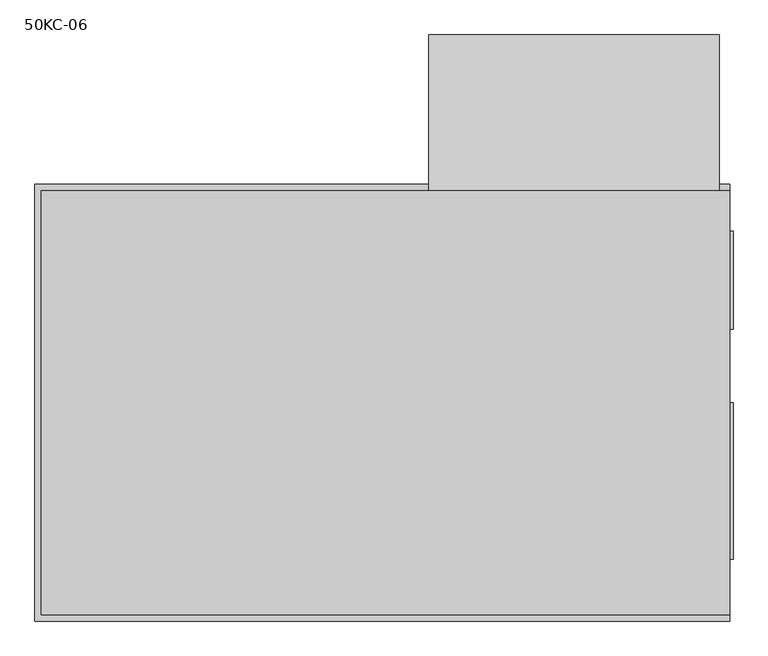
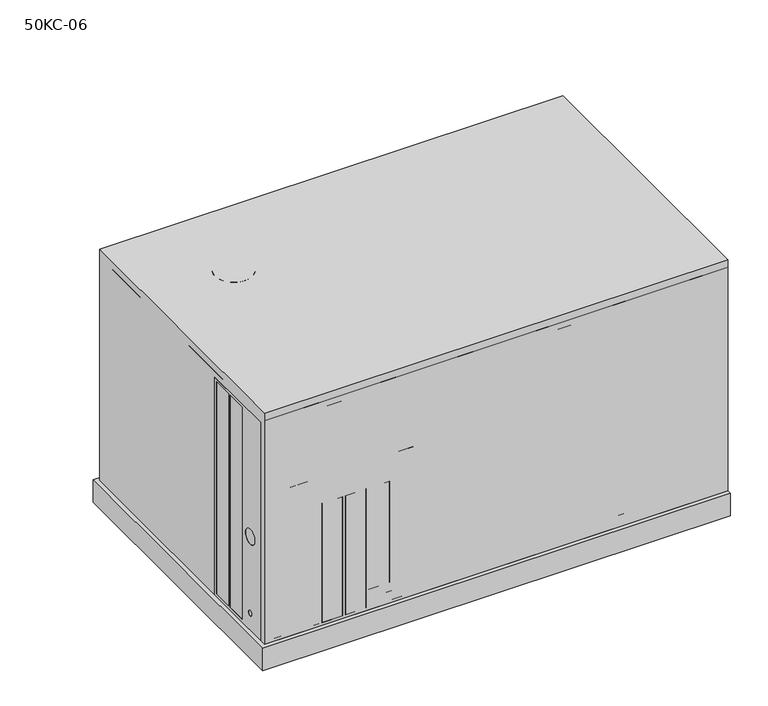
"""IFC4 building model written with IfcOpenShell, lengths in millimetres: proxy geometry, AHU-Rooftop-Carrier-Cooling_&_Elec_Heating-3-5_ton : 50KC-06."""

from ifc_helpers import new_model, si_unit, point, frame, frame_2d, origin, origin_with_axes, place, context, project, spatial, polyline, circle_curve, trimmed, segment, composite_curve, outline, extrude, faceted_brep, source, transform, mapped, element, save
from ifc_brep_helpers import plane_surface, cylinder_surface, revolved_surface, advanced_brep


def proxy_50kc_06_755dc8fb(model_context):
    return source(origin(), model_context, "Body", "SolidModel", [
        extrude(outline(polyline([(-547.6875, 1025.525), (-228.6, 1025.525), (-228.6, 95.25), (-547.6875, 95.25), (-547.6875, 1025.525)]), holes=[polyline([(-323.85, 1012.825), (-323.85, 107.95), (-241.3, 107.95), (-241.3, 1012.825), (-323.85, 1012.825)]), polyline([(-419.1, 1012.825), (-419.1, 107.95), (-336.55, 107.95), (-336.55, 1012.825), (-419.1, 1012.825)]), composite_curve([segment(trimmed(circle_curve(frame_2d((-476.25, 495.3)), 31.75), [point((-508.0, 495.3))], [point((-444.5, 495.3))], True, "CARTESIAN"), True, "CONTINUOUS"), segment(trimmed(circle_curve(frame_2d((-476.25, 495.3)), 31.75), [point((-444.5, 495.3))], [point((-508.0, 495.3))], True, "CARTESIAN"), True, "CONTINUOUS")], self_intersect=False), composite_curve([segment(trimmed(circle_curve(frame_2d((-476.25, 168.275)), 11.1125), [point((-487.3625, 168.275))], [point((-465.1375, 168.275))], True, "CARTESIAN"), True, "CONTINUOUS"), segment(trimmed(circle_curve(frame_2d((-476.25, 168.275)), 11.1125), [point((-465.1375, 168.275))], [point((-487.3625, 168.275))], True, "CARTESIAN"), True, "CONTINUOUS")], self_intersect=False)]), frame((-927.1, 0.0, 0.0), z_axis=(1.0, 0.0, 0.0), x_axis=(0.0, 1.0, 0.0)), (0.0, 0.0, 1.0), 3.175),
        advanced_brep(
        [(941.3875, 573.0875, 1025.525), (-436.5625, 573.0875, 1025.525), (-436.5625, 534.9875, 1025.525), (-885.825, 534.9875, 1025.525), (-885.825, -215.9, 1025.525), (-923.925, -215.9, 1025.525), (-923.925, -573.0875, 1025.525), (941.3875, -573.0875, 1025.525), (-883.285, 532.4475, 1025.525), (-436.5625, 532.4475, 1025.525), (-436.5625, -215.9, 1025.525), (-883.285, -215.9, 1025.525), (941.3875, 573.0875, 95.25), (941.3875, -573.0875, 95.25), (-923.925, -573.0875, 95.25), (-923.925, -215.9, 95.25), (-885.825, -215.9, 95.25), (-885.825, 534.9875, 95.25), (-436.5625, 534.9875, 95.25), (-436.5625, 573.0875, 95.25), (-883.285, 532.4475, 95.25), (-883.285, -215.9, 95.25), (-436.5625, -215.9, 95.25), (-436.5625, 532.4475, 95.25), (-923.925, -508.0, 495.3), (-923.925, -444.5, 495.3), (-923.925, -487.3625, 168.275), (-923.925, -465.1375, 168.275), (941.3875, 88.9, 194.1909375), (941.3875, 88.9, 161.4090625), (919.1625, 88.9, 161.4090625), (919.1625, 88.9, 194.1909375), (-914.4, -508.0, 495.3), (-914.4, -444.5, 495.3), (-914.4, -487.3625, 168.275), (-914.4, -465.1375, 168.275)],
        [
            (0, 1),
            (1, 2),
            (2, 3),
            (3, 4),
            (4, 5),
            (5, 6),
            (6, 7),
            (7, 0),
            (8, 9),
            (9, 10),
            (10, 11),
            (11, 8),
            (12, 13),
            (13, 14),
            (14, 15),
            (15, 16),
            (16, 17),
            (17, 18),
            (18, 19),
            (19, 12),
            (20, 21),
            (21, 22),
            (22, 23),
            (23, 20),
            (0, 12),
            (19, 1),
            (5, 15),
            (14, 6),
            (24, 25, circle_curve(frame((-923.925, -476.25, 495.3), z_axis=(1.0, 0.0, 0.0), x_axis=(0.0, 1.0, 0.0)), 31.75)),
            (25, 24, circle_curve(frame((-923.925, -476.25, 495.3), z_axis=(1.0, 0.0, 0.0), x_axis=(0.0, 1.0, 0.0)), 31.75)),
            (26, 27, circle_curve(frame((-923.925, -476.25, 168.275), z_axis=(1.0, 0.0, 0.0), x_axis=(0.0, 1.0, 0.0)), 11.1125)),
            (27, 26, circle_curve(frame((-923.925, -476.25, 168.275), z_axis=(1.0, 0.0, 0.0), x_axis=(0.0, 1.0, 0.0)), 11.1125)),
            (13, 7),
            (28, 29, circle_curve(frame((941.3875, 88.9, 177.8), z_axis=(-1.0, 0.0, 0.0), x_axis=(0.0, 0.0, 1.0)), 16.3909375)),
            (29, 28, circle_curve(frame((941.3875, 88.9, 177.8), z_axis=(-1.0, 0.0, 0.0), x_axis=(0.0, 0.0, 1.0)), 16.3909375)),
            (18, 2),
            (17, 3),
            (16, 4),
            (30, 31, circle_curve(frame((919.1625, 88.9, 177.8), z_axis=(1.0, 0.0, 0.0), x_axis=(0.0, 0.0, 1.0)), 16.3909375)),
            (31, 30, circle_curve(frame((919.1625, 88.9, 177.8), z_axis=(1.0, 0.0, 0.0), x_axis=(0.0, 0.0, 1.0)), 16.3909375)),
            (30, 29),
            (28, 31),
            (32, 33, circle_curve(frame((-914.4, -476.25, 495.3), z_axis=(-1.0, 0.0, 0.0), x_axis=(0.0, 1.0, 0.0)), 31.75)),
            (33, 32, circle_curve(frame((-914.4, -476.25, 495.3), z_axis=(-1.0, 0.0, 0.0), x_axis=(0.0, 1.0, 0.0)), 31.75)),
            (34, 35, circle_curve(frame((-914.4, -476.25, 168.275), z_axis=(-1.0, 0.0, 0.0), x_axis=(0.0, 1.0, 0.0)), 11.1125)),
            (35, 34, circle_curve(frame((-914.4, -476.25, 168.275), z_axis=(-1.0, 0.0, 0.0), x_axis=(0.0, 1.0, 0.0)), 11.1125)),
            (33, 25),
            (24, 32),
            (35, 27),
            (26, 34),
            (8, 20),
            (23, 9),
            (22, 10),
            (21, 11),
        ],
        [
            plane_surface(frame((-466.3462048, 573.0875, 1025.525), z_axis=(0.0, 0.0, 1.0), x_axis=(-1.0, 0.0, 0.0))),
            plane_surface(frame((-466.3462048, 573.0875, 95.25), z_axis=(0.0, 0.0, -1.0), x_axis=(1.0, 0.0, 0.0))),
            plane_surface(frame((941.3875, 573.0875, 1025.525), z_axis=(0.0, 1.0, 0.0), x_axis=(0.0, 0.0, -1.0))),
            plane_surface(frame((-923.925, -215.9, 1025.525), z_axis=(-1.0, 0.0, 0.0), x_axis=(0.0, 0.0, -1.0))),
            plane_surface(frame((-923.925, -573.0875, 1025.525), z_axis=(0.0, -1.0, 0.0), x_axis=(0.0, 0.0, -1.0))),
            plane_surface(frame((941.3875, -573.0875, 1025.525), z_axis=(1.0, 0.0, 0.0), x_axis=(0.0, 0.0, -1.0))),
            plane_surface(frame((-436.5625, 573.0875, 1025.525), z_axis=(-1.0, 0.0, 0.0), x_axis=(0.0, 0.0, -1.0))),
            plane_surface(frame((-436.5625, 534.9875, 1025.525), z_axis=(0.0, 1.0, 0.0), x_axis=(0.0, 0.0, -1.0))),
            plane_surface(frame((-885.825, 534.9875, 1025.525), z_axis=(-1.0, 0.0, 0.0), x_axis=(0.0, 0.0, -1.0))),
            plane_surface(frame((-885.825, -215.9, 1025.525), z_axis=(0.0, 1.0, 0.0), x_axis=(0.0, 0.0, -1.0))),
            plane_surface(frame((919.1625, 88.9, 177.8), z_axis=(1.0, 0.0, 0.0), x_axis=(0.0, 1.0, 0.0))),
            revolved_surface(polyline([(941.3875, 88.9, 194.19093750000002), (919.1625, 88.9, 194.19093750000002)]), (944.5625, 88.9, 177.8), (1.0, 0.0, 0.0)),
            plane_surface(frame((-914.4, -444.5, 495.3), z_axis=(-1.0, 0.0, 0.0), x_axis=(0.0, 0.0, 1.0))),
            revolved_surface(polyline([(-914.4, -444.5, 495.3), (-923.925, -444.5, 495.3)]), (-927.1, -476.25, 495.3), (1.0, 0.0, 0.0)),
            revolved_surface(polyline([(-914.4, -465.1375, 168.275), (-923.925, -465.1375, 168.275)]), (-927.1, -476.25, 168.275), (1.0, 0.0, 0.0)),
            plane_surface(frame((-883.285, 532.4475, 1025.525), z_axis=(0.0, -1.0, 0.0), x_axis=(0.0, 0.0, -1.0))),
            plane_surface(frame((-436.5625, 532.4475, 1025.525), z_axis=(-1.0, 0.0, 0.0), x_axis=(0.0, 0.0, -1.0))),
            plane_surface(frame((-436.5625, -215.9, 1025.525), z_axis=(0.0, 1.0, 0.0), x_axis=(0.0, 0.0, -1.0))),
            plane_surface(frame((-883.285, -215.9, 1025.525), z_axis=(1.0, 0.0, 0.0), x_axis=(0.0, 0.0, -1.0))),
        ],
        [
            (0, [[1, 2, 3, 4, 5, 6, 7, 8], [9, 10, 11, 12]]),
            (1, [[13, 14, 15, 16, 17, 18, 19, 20], [21, 22, 23, 24]]),
            (2, [[-1, 25, -20, 26]]),
            (3, [[-6, 27, -15, 28], [29, 30], [31, 32]]),
            (4, [[-7, -28, -14, 33]]),
            (5, [[-8, -33, -13, -25], [34, 35]]),
            (6, [[-2, -26, -19, 36]]),
            (7, [[-3, -36, -18, 37]]),
            (8, [[-4, -37, -17, 38]]),
            (9, [[-5, -38, -16, -27]]),
            (10, [[39, 40]]),
            (11, [[-39, 41, -34, 42]]),
            (11, [[-40, -42, -35, -41]]),
            (12, [[43, 44]]),
            (12, [[45, 46]]),
            (13, [[-44, 47, -29, 48]]),
            (13, [[-43, -48, -30, -47]]),
            (14, [[-46, 49, -31, 50]]),
            (14, [[-45, -50, -32, -49]]),
            (15, [[-9, 51, -24, 52]]),
            (16, [[-10, -52, -23, 53]]),
            (17, [[-11, -53, -22, 54]]),
            (18, [[-12, -54, -21, -51]]),
        ],
    ),
        faceted_brep([(-898.525, 573.0875, 1025.525), (-923.925, 573.0875, 1025.525), (-923.925, 547.6875, 1025.525), (-898.525, 547.6875, 1025.525), (-898.525, 573.0875, 95.25), (-898.525, 547.6875, 95.25), (-923.925, 547.6875, 95.25), (-923.925, 573.0875, 95.25)], [[[0, 1, 2, 3]], [[4, 5, 6, 7]], [[1, 0, 4, 7]], [[2, 1, 7, 6]], [[3, 2, 6, 5]], [[0, 3, 5, 4]]]),
        extrude(outline(polyline([(941.3875, 466.725), (954.0875, 466.725), (954.0875, 200.025), (941.3875, 200.025), (941.3875, 466.725)])), frame((0.0, 0.0, 155.575), z_axis=(0.0, 0.0, 1.0), x_axis=(1.0, 0.0, 0.0)), (0.0, 0.0, 1.0), 638.175),
        extrude(outline(polyline([(941.3875, 0.0), (954.0875, 0.0), (954.0875, -425.45), (941.3875, -425.45), (941.3875, 0.0)])), frame((0.0, 0.0, 155.575), z_axis=(0.0, 0.0, 1.0), x_axis=(1.0, 0.0, 0.0)), (0.0, 0.0, 1.0), 288.925),
        extrude(outline(polyline([(944.5625, 576.2625), (944.5625, -576.2625), (-927.1, -576.2625), (-927.1, 576.2625), (944.5625, 576.2625)])), frame((0.0, 0.0, 95.25), z_axis=(0.0, 0.0, 1.0), x_axis=(1.0, 0.0, 0.0)), (0.0, 0.0, 1.0), 987.425),
        extrude(outline(polyline([(-944.5625, 593.725), (944.5625, 593.725), (944.5625, -593.725), (-944.5625, -593.725), (-944.5625, 593.725)])), origin_with_axes(), (0.0, 0.0, 1.0), 95.25),
        extrude(outline(polyline([(21.43125, -576.2625), (-3.96875, -576.2625), (-3.96875, 576.2625), (21.43125, 576.2625), (21.43125, -576.2625)])), frame((0.0, 0.0, 1050.925), z_axis=(0.0, 0.0, 1.0), x_axis=(1.0, 0.0, 0.0)), (0.0, 0.0, 1.0), 12.7),
        extrude(outline(polyline([(1025.525, -411.1625), (95.25, -411.1625), (95.25, 101.6), (1025.525, 101.6), (1025.525, -411.1625)]), holes=[polyline([(177.8, -202.40625), (177.8, -107.15625), (146.05, -107.15625), (146.05, -202.40625), (177.8, -202.40625)])]), frame((0.0, 573.0875, 0.0), z_axis=(0.0, 1.0, 0.0), x_axis=(0.0, 0.0, 1.0)), (0.0, 0.0, 1.0), 3.175),
        extrude(outline(polyline([(915.9875, 573.0875), (127.0, 573.0875), (127.0, 576.2625), (915.9875, 576.2625), (915.9875, 573.0875)])), frame((0.0, 0.0, 546.1), z_axis=(0.0, 0.0, 1.0), x_axis=(1.0, 0.0, 0.0)), (0.0, 0.0, 1.0), 479.425),
        extrude(outline(polyline([(915.9875, 573.0875), (127.0, 573.0875), (127.0, 576.2625), (915.9875, 576.2625), (915.9875, 573.0875)])), frame((0.0, 0.0, 95.25), z_axis=(0.0, 0.0, 1.0), x_axis=(1.0, 0.0, 0.0)), (0.0, 0.0, 1.0), 444.5),
        extrude(outline(polyline([(-923.925, -336.55), (-923.925, -419.1), (-927.1, -419.1), (-927.1, -336.55), (-923.925, -336.55)])), frame((0.0, 0.0, 107.95), z_axis=(0.0, 0.0, 1.0), x_axis=(1.0, 0.0, 0.0)), (0.0, 0.0, 1.0), 904.875),
        extrude(outline(polyline([(-923.925, -241.3), (-923.925, -323.85), (-927.1, -323.85), (-927.1, -241.3), (-923.925, -241.3)])), frame((0.0, 0.0, 107.95), z_axis=(0.0, 0.0, 1.0), x_axis=(1.0, 0.0, 0.0)), (0.0, 0.0, 1.0), 904.875),
        extrude(outline(polyline([(-803.275, -576.2625), (-885.825, -576.2625), (-885.825, -573.0875), (-803.275, -573.0875), (-803.275, -576.2625)])), frame((0.0, 0.0, 107.95), z_axis=(0.0, 0.0, 1.0), x_axis=(1.0, 0.0, 0.0)), (0.0, 0.0, 1.0), 622.3),
        extrude(outline(polyline([(-708.025, -576.2625), (-790.575, -576.2625), (-790.575, -573.0875), (-708.025, -573.0875), (-708.025, -576.2625)])), frame((0.0, 0.0, 107.95), z_axis=(0.0, 0.0, 1.0), x_axis=(1.0, 0.0, 0.0)), (0.0, 0.0, 1.0), 622.3),
        extrude(outline(polyline([(-612.775, -576.2625), (-695.325, -576.2625), (-695.325, -573.0875), (-612.775, -573.0875), (-612.775, -576.2625)])), frame((0.0, 0.0, 107.95), z_axis=(0.0, 0.0, 1.0), x_axis=(1.0, 0.0, 0.0)), (0.0, 0.0, 1.0), 508.0),
        extrude(outline(polyline([(-517.525, -576.2625), (-600.075, -576.2625), (-600.075, -573.0875), (-517.525, -573.0875), (-517.525, -576.2625)])), frame((0.0, 0.0, 107.95), z_axis=(0.0, 0.0, 1.0), x_axis=(1.0, 0.0, 0.0)), (0.0, 0.0, 1.0), 508.0),
        extrude(outline(polyline([(-422.275, -576.2625), (-504.825, -576.2625), (-504.825, -573.0875), (-422.275, -573.0875), (-422.275, -576.2625)])), frame((0.0, 0.0, 184.15), z_axis=(0.0, 0.0, 1.0), x_axis=(1.0, 0.0, 0.0)), (0.0, 0.0, 1.0), 431.8),
        extrude(outline(polyline([(-327.025, -576.2625), (-409.575, -576.2625), (-409.575, -573.0875), (-327.025, -573.0875), (-327.025, -576.2625)])), frame((0.0, 0.0, 107.95), z_axis=(0.0, 0.0, 1.0), x_axis=(1.0, 0.0, 0.0)), (0.0, 0.0, 1.0), 622.3),
        extrude(outline(polyline([(1025.525, 915.9875), (1025.525, 34.13125), (95.25, 34.13125), (95.25, 915.9875), (1025.525, 915.9875)]), holes=[polyline([(177.8, 522.684375), (146.05, 522.684375), (146.05, 427.434375), (177.8, 427.434375), (177.8, 522.684375)])]), frame((0.0, -576.2625, 0.0), z_axis=(0.0, 1.0, 0.0), x_axis=(0.0, 0.0, 1.0)), (0.0, 0.0, 1.0), 3.175),
        extrude(outline(polyline([(1025.525, -16.66875), (1025.525, -898.525), (95.25, -898.525), (95.25, -16.66875), (1025.525, -16.66875)]), holes=[polyline([(177.8, -415.925), (146.05, -415.925), (146.05, -511.175), (177.8, -511.175), (177.8, -415.925)]), polyline([(730.25, -803.275), (107.95, -803.275), (107.95, -885.825), (730.25, -885.825), (730.25, -803.275)]), polyline([(730.25, -708.025), (107.95, -708.025), (107.95, -790.575), (730.25, -790.575), (730.25, -708.025)]), polyline([(615.95, -612.775), (107.95, -612.775), (107.95, -695.325), (615.95, -695.325), (615.95, -612.775)]), polyline([(615.95, -517.525), (107.95, -517.525), (107.95, -600.075), (615.95, -600.075), (615.95, -517.525)]), polyline([(615.95, -422.275), (184.15, -422.275), (184.15, -504.825), (615.95, -504.825), (615.95, -422.275)]), polyline([(730.25, -327.025), (107.95, -327.025), (107.95, -409.575), (730.25, -409.575), (730.25, -327.025)])]), frame((0.0, -576.2625, 0.0), z_axis=(0.0, 1.0, 0.0), x_axis=(0.0, 0.0, 1.0)), (0.0, 0.0, 1.0), 3.175),
        extrude(outline(polyline([(1000.125, 464.451767), (997.9196681, 451.9447085), (947.8914343, 460.7660359), (709.1843069, 119.8569277), (573.0875, 107.95), (573.0875, 539.75), (1000.125, 464.451767)])), frame((127.0, 0.0, 0.0), z_axis=(1.0, 0.0, 0.0), x_axis=(0.0, 1.0, 0.0)), (0.0, 0.0, 1.0), 788.9875),
        advanced_brep(
        [(-584.2, 233.3625, 1082.675), (-660.4, 233.3625, 1082.675), (-508.0, 233.3625, 1082.675), (-660.4, 233.3625, 1079.5), (-508.0, 233.3625, 1079.5), (-863.6, 233.3625, 1050.925), (-304.8, 233.3625, 1050.925), (-584.2, 233.3625, 1050.925)],
        [
            (0, 1),
            (1, 2, circle_curve(frame((-584.2, 233.3625, 1082.675), z_axis=(0.0, 0.0, 1.0), x_axis=(-1.0, 0.0, 0.0)), 76.2)),
            (2, 0),
            (2, 1, circle_curve(frame((-584.2, 233.3625, 1082.675), z_axis=(0.0, 0.0, 1.0), x_axis=(-1.0, 0.0, 0.0)), 76.2)),
            (1, 3),
            (3, 4, circle_curve(frame((-584.2, 233.3625, 1079.5), z_axis=(0.0, 0.0, 1.0), x_axis=(-1.0, 0.0, 0.0)), 76.2)),
            (4, 2),
            (4, 3, circle_curve(frame((-584.2, 233.3625, 1079.5), z_axis=(0.0, 0.0, 1.0), x_axis=(-1.0, 0.0, 0.0)), 76.2)),
            (3, 5),
            (5, 6, circle_curve(frame((-584.2, 233.3625, 1050.925), z_axis=(0.0, 0.0, 1.0), x_axis=(-1.0, 0.0, 0.0)), 279.4)),
            (6, 4),
            (6, 5, circle_curve(frame((-584.2, 233.3625, 1050.925), z_axis=(0.0, 0.0, 1.0), x_axis=(-1.0, 0.0, 0.0)), 279.4)),
            (5, 7),
            (7, 6),
        ],
        [
            plane_surface(frame((-584.2, 233.3625, 1082.675), z_axis=(0.0, 0.0, 1.0), x_axis=(-1.0, 0.0, 0.0))),
            cylinder_surface(frame((-584.2, 233.3625, 1654.166912), z_axis=(0.0, 0.0, 1.0), x_axis=(-1.0, 0.0, 0.0)), 76.2),
            revolved_surface(polyline([(-863.6, 233.3625, 1050.925), (-660.4, 233.3625, 1079.5)]), (-584.2, 233.3625, 1654.166912), (0.0, 0.0, 1.0)),
            plane_surface(frame((-584.2, 233.3625, 1050.925), z_axis=(0.0, 0.0, -1.0), x_axis=(-1.0, 0.0, 0.0))),
        ],
        [
            (0, [[1, 2, 3]]),
            (0, [[-3, 4, -1]]),
            (1, [[-2, 5, 6, 7]]),
            (1, [[-4, -7, 8, -5]]),
            (2, [[-6, 9, 10, 11]]),
            (2, [[-8, -11, 12, -9]]),
            (3, [[-10, 13, 14]]),
            (3, [[-12, -14, -13]]),
        ],
    ),
        extrude(outline(polyline([(944.5625, 576.2625), (944.5625, -576.2625), (-927.1, -576.2625), (-927.1, 576.2625), (944.5625, 576.2625)])), frame((0.0, 0.0, 1025.525), z_axis=(0.0, 0.0, 1.0), x_axis=(1.0, 0.0, 0.0)), (0.0, 0.0, 1.0), 25.4),
        extrude(outline(polyline([(944.5625, 593.725), (944.5625, -593.725), (-944.5625, -593.725), (-944.5625, 593.725), (944.5625, 593.725)]), holes=[polyline([(877.8875, 527.05), (-877.8875, 527.05), (-877.8875, -527.05), (877.8875, -527.05), (877.8875, 527.05)])]), origin_with_axes(), (0.0, 0.0, 1.0), 95.25),
    ])


if __name__ == "__main__":
    model = new_model("IFC4")
    model_context = context("Model", 3, world=origin())
    ifc_project = project(units=[si_unit("LENGTHUNIT", "METRE", prefix="MILLI")], contexts=[model_context])
    site = spatial("IfcSite", under=ifc_project)
    building = spatial("IfcBuilding", under=site)
    placement = place(None, origin())
    proxy_50kc_06_shape = proxy_50kc_06_755dc8fb(model_context)
    element("IfcBuildingElementProxy", 1, Name="AHU-Rooftop-Carrier-Cooling_&_Elec_Heating-3-5_ton : 50KC-06", ObjectType="AHU-Rooftop-Carrier-Cooling_&_Elec_Heating-3-5_ton : 50KC-06", at=placement, inside=building, context=model_context, shape_type="MappedRepresentation", body=[
        mapped(proxy_50kc_06_shape, transform((0.0, 0.0, 0.0), x_axis=(1.0, 0.0, 0.0), y_axis=(0.0, 1.0, 0.0), z_axis=(0.0, 0.0, 1.0))),
    ])
    save(model, "model.ifc")

# Revit data of these elements
# Type "AHU-Rooftop-Carrier-Cooling_&_Elec_Heating-3-5_ton : 50KC-06"
#   URL = "www.carrier.com"
#   Model = "50KC-06"
#   Manufacturer = "Carrier Corporation"
#   Assembly Code = "D3050200"
#   Width = 3' - 10 3/4"
#   Voltage [instance default] = 240 V
#   SA Z Offset [instance default] = 0' - 2 3/8"
#   SA Y Offset [instance default] = 0' - 6 5/8"
#   SA X Offset [instance default] = 0' - 0"
#   SA Width [instance default] = 16 3/4"
#   SA Height [instance default] = 11 3/8"
#   RA Z Offset [instance default] = 0' - 2 3/8"
#   RA Y Offset [instance default] = 2' - 7 1/4"
#   RA X Offset [instance default] = 0' - 0"
#   RA Width [instance default] = 10 1/2"
#   RA Height [instance default] = 25 1/8"
#   Power Factor [instance default] = 0.8
#   Lid Lap = 0' - 0 1/8"
#   Lid Height = 0' - 1"
#   Length 9 [instance default] = 0' - 0"
#   Length 8 [instance default] = 0' - 0"
#   Length 7 [instance default] = 0' - 0"
#   Length 6 [instance default] = 0' - 0"
#   Length 5 [instance default] = 0' - 0"
#   Length 4 = 0' - 1"
#   Length 3 [instance default] = 1' - 4"
#   Length 2 = 1' - 1 1/2"
#   Length 1 [instance default] = 0' - 0"
#   Length = 6' - 2 3/8"
#   Height = 3' - 5 3/8"
#   Handle Width = 0' - 3 3/4"
#   Handle Height = 0' - 1 1/4"
#   Grille Radius = 0' - 11"
#   Grille Plate Radius = 0' - 3"
#   Frame Width = 0' - 1"
#   Fan Height = 0' - 1 1/4"
#   Electrical Panel Length = 1' - 2 7/8"
#   Economizer Width = 1' - 4"
#   Economizer Offset = 1' - 9 1/4"
#   Economizer Length = 2' - 7 1/16"
#   Economizer Height = 1' - 5"
#   Drain Z Offset [instance default] = 0' - 3 1/4"
#   Drain Y Offset [instance default] = 2' - 2 7/8"
#   Drain X Offset [instance default] = 0' - 0"
#   Drain Radius [instance default] = 3/8"
#   Drain Hole Radius [instance default] = 0' - 0.64531"
#   Curb Width = 0' - 2 5/8"
#   Curb Height = 0' - 3 3/4"
#   Clearance Top [instance default] = 5' - 0"
#   Clearance Right [instance default] = 3' - 0"
#   Clearance Left [instance default] = 4' - 0"
#   Clearance Front [instance default] = 4' - 0"
#   Clearance Back [instance default] = 3' - 6"
#   Apparent Load [instance default] = 0 VA
#   Angle 3 [instance default] = 270.00°
#   Angle 2 [instance default] = 90.00°
#   Angle 1 [instance default] = 90.00°
#   Vertical Supply Air [instance default] = no
#   Vertical Return Air [instance default] = no
#   Standard Drain [instance default] = yes
#   Roof Curb [instance default] = yes
#   Number of Poles [instance default] = 3
#   Horizontal Supply Air [instance default] = yes
#   Horizontal Return Air [instance default] = yes
#   Economizer [instance default] = yes
#   Clearance Zones [instance default] = no
#   Alternate Drain [instance default] = no
#   Load Classification = HVAC
#   Highlight Material = Paint - Carrier - Black
#   Grille Material = Metal - Carrier - Grille 2
#   Fan Material = Metal - Carrier - Grille
#   Curb Material = Metal - Carrier - Steel
#   Clearance Material = Clearance Zone
#   Body Material = RTU'S - SIZE AND LOCATION T.B.D.
# Element 1 (IfcBuildingElementProxy, "AHU-Rooftop-Carrier-Cooling_&_Elec_Heating-3-5_ton : 50KC-06")
#   Materials on its faces: "RTU'S - SIZE AND LOCATION T.B.D.", "Metal - Carrier - Grille 2", "Metal - Carrier - Steel", "Paint - Carrier - Black", "Metal - Carrier - Grille"
# Materials
#   "Paint - Carrier - Black": class "Miscellaneous", colour RGB 46 46 46, transparency 0
#   "Metal - Carrier - Grille 2": class "Miscellaneous", colour RGB 182 199 209, transparency 0
#   "Metal - Carrier - Grille": class "Miscellaneous", colour RGB 115 113 111, transparency 0
#   "Metal - Carrier - Steel": class "Miscellaneous", colour RGB 192 192 192, transparency 0
#   "Clearance Zone": class "Glass", colour RGB 255 0 0, transparency 0.85
#   "RTU'S - SIZE AND LOCATION T.B.D.": class "Miscellaneous", colour RGB 182 199 209, transparency 0, Cost = 0
